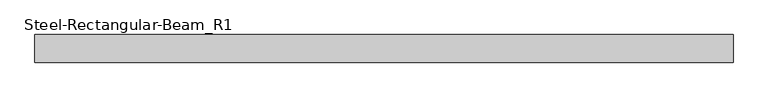
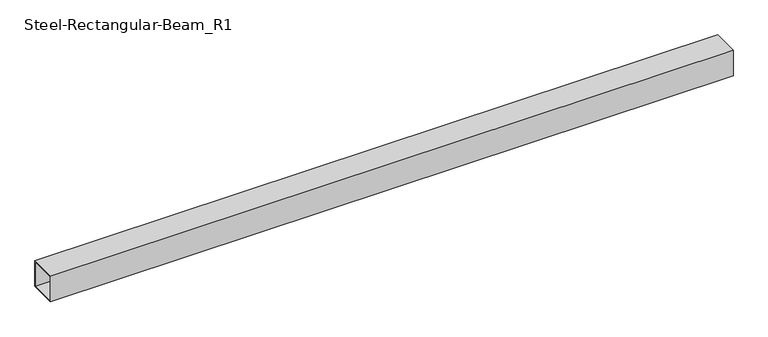
"""IFC4 building model written with IfcOpenShell, lengths in millimetres: beam geometry, Steel-Rectangular-Beam_R1 : BM125_RT-100x100x4.0_RB1."""

from ifc_helpers import new_model, si_unit, frame, origin, place, context, project, spatial, polyline, outline, extrude, source, transform, mapped, element, save


def steel_rectangular_beam_r1_1c4b02f8(model_context):
    return source(origin(), model_context, "Body", "SweptSolid", [
        extrude(outline(polyline([(-50.0, 50.0), (50.0, 50.0), (50.0, -50.0), (-50.0, -50.0), (-50.0, 50.0)]), holes=[polyline([(46.0, -46.0), (46.0, 46.0), (-46.0, 46.0), (-46.0, -46.0), (46.0, -46.0)])]), frame((-2955.3, 0.0, 0.0), z_axis=(1.0, 0.0, 0.0), x_axis=(0.0, 1.0, 0.0)), (0.0, 0.0, 1.0), 2529.1991316),
        extrude(outline(polyline([(-50.0, 50.0), (50.0, 50.0), (50.0, -50.0), (-50.0, -50.0), (-50.0, 50.0)]), holes=[polyline([(46.0, -46.0), (46.0, 46.0), (-46.0, 46.0), (-46.0, -46.0), (46.0, -46.0)])]), frame((-2955.3, 0.0, 0.0), z_axis=(1.0, 0.0, 0.0), x_axis=(0.0, 1.0, 0.0)), (0.0, 0.0, 1.0), 2529.1991316),
        extrude(outline(polyline([(-50.0, 50.0), (50.0, 50.0), (50.0, -50.0), (-50.0, -50.0), (-50.0, 50.0)]), holes=[polyline([(46.0, -46.0), (46.0, 46.0), (-46.0, 46.0), (-46.0, -46.0), (46.0, -46.0)])]), frame((-2955.3, 0.0, 0.0), z_axis=(1.0, 0.0, 0.0), x_axis=(0.0, 1.0, 0.0)), (0.0, 0.0, 1.0), 2529.1991316),
        extrude(outline(polyline([(-50.0, 50.0), (50.0, 50.0), (50.0, -50.0), (-50.0, -50.0), (-50.0, 50.0)]), holes=[polyline([(46.0, -46.0), (46.0, 46.0), (-46.0, 46.0), (-46.0, -46.0), (46.0, -46.0)])]), frame((-2955.3, 0.0, 0.0), z_axis=(1.0, 0.0, 0.0), x_axis=(0.0, 1.0, 0.0)), (0.0, 0.0, 1.0), 2529.1991316),
    ])


if __name__ == "__main__":
    model = new_model("IFC4")
    model_context = context("Model", 3, world=origin())
    ifc_project = project(units=[si_unit("LENGTHUNIT", "METRE", prefix="MILLI")], contexts=[model_context])
    site = spatial("IfcSite", under=ifc_project)
    building = spatial("IfcBuilding", under=site)
    placement = place(None, origin())
    steel_rectangular_beam_r1_shape = steel_rectangular_beam_r1_1c4b02f8(model_context)
    element("IfcBeam", 1, ObjectType="Steel-Rectangular-Beam_R1 : BM125_RT-100x100x4.0_RB1", at=placement, inside=building, context=model_context, shape_type="MappedRepresentation", body=[
        mapped(steel_rectangular_beam_r1_shape, transform((0.0, 0.0, 0.0), x_axis=(1.0, 0.0, 0.0), y_axis=(0.0, 1.0, 0.0), z_axis=(0.0, 0.0, 1.0))),
    ])
    save(model, "model.ifc")

# Revit data of these elements
# Type "Steel-Rectangular-Beam_R1 : BM125_RT-100x100x4.0_RB1"
#   SteelWeight = "Light"
#   t = 4 mm
#   Mass per Unit Length = 11.70 kg/m
#   Surface Area = 0.40 m²/m
#   Section Area = 14.95 cm²
#   Length [instance default] = 3000 mm
#   H = 100 mm
#   B = 100 mm
#   hec_material4 [instance default] = none
#   hec_material3 [instance default] = none
#   hec_material2 [instance default] = none
#   hec_material1 [instance default] = none
#   Structural Material [instance default] = none
